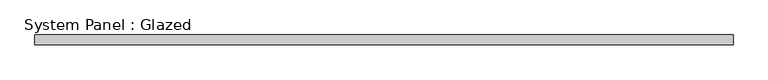
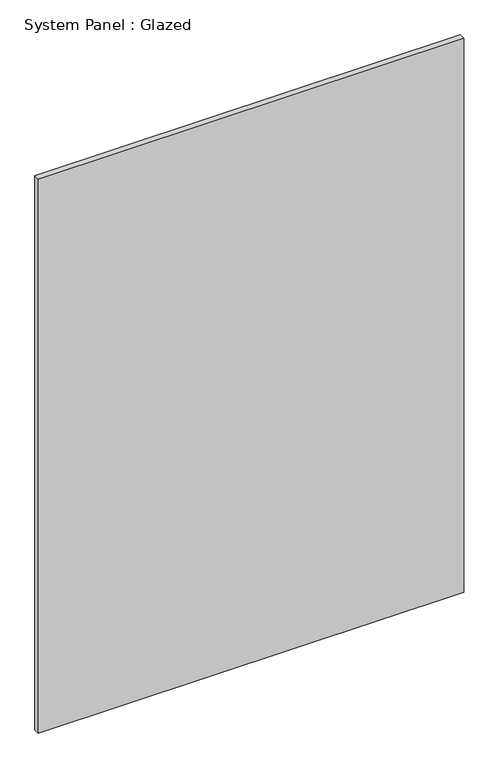
"""IFC4 building model written with IfcOpenShell, lengths in millimetres: plate geometry, System Panel : Glazed."""

import ifcopenshell
import ifcopenshell.guid

model = None  # the IFC model being written
_history = None  # IfcOwnerHistory: only IFC2X3 demands one
_inside = {}  # id of a spatial element -> (the spatial element, [elements in it])
_under = {}  # id of a project, library or spatial element -> (it, [spatial elements below it])
_declared = {}  # id of a project -> (the project, [libraries it declares])
_typed = {}  # id of a type object -> (the type object, [elements of that type])
_made_of = {}  # id of a material, layer set ... -> (it, [elements and type objects made of it])


def new_model(schema):
    """Start an empty IFC model of exactly this schema.

    Asked for "IFC4X3", IfcOpenShell would pick the latest addendum, in which some entities
    have other attributes; the version numbers below select the first issue.
    IFC2X3 requires an IfcOwnerHistory on every rooted entity: one is made here for all.
    """
    global model, _history
    if schema == "IFC4X3":
        model = ifcopenshell.file(schema_version=(4, 3, 0, 0))
    else:
        model = ifcopenshell.file(schema=schema)
    _inside.clear()
    _under.clear()
    _declared.clear()
    _typed.clear()
    _made_of.clear()
    _history = None
    if model.schema == "IFC2X3":
        org = make("IfcOrganization", Name="unknown")
        user = make(
            "IfcPersonAndOrganization",
            ThePerson=make("IfcPerson", FamilyName="unknown"),
            TheOrganization=org,
        )
        app = make(
            "IfcApplication",
            ApplicationDeveloper=org,
            Version="unknown",
            ApplicationFullName="unknown",
            ApplicationIdentifier="unknown",
        )
        _history = make(
            "IfcOwnerHistory",
            OwningUser=user,
            OwningApplication=app,
            ChangeAction="ADDED",
            CreationDate=0,
        )
    return model


def make(cls, **values):
    """One entity of the class cls with the attributes given. An attribute that is None is left unset."""
    return model.create_entity(
        cls, **{name: value for name, value in values.items() if value is not None}
    )


def rooted(cls, **values):
    """An entity with a GlobalId (a new one), such as an element, a storey or a relation."""
    return make(cls, GlobalId=ifcopenshell.guid.new(), OwnerHistory=_history, **values)


def si_unit(unit_type, name, prefix=None):
    """IfcSIUnit, for example si_unit("LENGTHUNIT", "METRE", prefix="MILLI")."""
    return make("IfcSIUnit", UnitType=unit_type, Prefix=prefix, Name=name)


def assignment(units):
    """IfcUnitAssignment: the units of a project."""
    return None if units is None else make("IfcUnitAssignment", Units=units)


def point(xyz):
    """IfcCartesianPoint."""
    return None if xyz is None else make("IfcCartesianPoint", Coordinates=xyz)


def direction(xyz):
    """IfcDirection."""
    return None if xyz is None else make("IfcDirection", DirectionRatios=xyz)


def frame(location, z_axis=None, x_axis=None):
    """IfcAxis2Placement3D, a coordinate frame: its origin and axes. An axis left out is left unset."""
    return make(
        "IfcAxis2Placement3D",
        Location=point(location),
        Axis=direction(z_axis),
        RefDirection=direction(x_axis),
    )


def origin():
    """The frame at (0, 0, 0) with its axes left unset."""
    return frame((0.0, 0.0, 0.0))


def origin_with_axes():
    """The frame at (0, 0, 0) with the z axis (0, 0, 1) and the x axis (1, 0, 0) written out."""
    return frame((0.0, 0.0, 0.0), z_axis=(0.0, 0.0, 1.0), x_axis=(1.0, 0.0, 0.0))


def place(relative_to, where):
    """IfcLocalPlacement: puts the frame where relative to a parent placement (None: the world)."""
    return make(
        "IfcLocalPlacement", PlacementRelTo=relative_to, RelativePlacement=where
    )


def context(
    kind, dimensions, precision=None, world=None, true_north=None, identifier=None
):
    """IfcGeometricRepresentationContext, for example the 3D "Model" context."""
    return make(
        "IfcGeometricRepresentationContext",
        ContextIdentifier=identifier,
        ContextType=kind,
        CoordinateSpaceDimension=dimensions,
        Precision=precision,
        WorldCoordinateSystem=world,
        TrueNorth=true_north,
    )


def project(units=None, contexts=None):
    """IfcProject with its units and contexts."""
    return rooted(
        "IfcProject",
        Name="project",
        RepresentationContexts=contexts,
        UnitsInContext=assignment(units),
    )


def spatial(cls, under=None, at=None, **own):
    """A site, building, storey or space (cls), placed at a placement, below another one or the project."""
    s = rooted(cls, ObjectPlacement=at, **own)
    if under is not None:
        _under.setdefault(under.id(), (under, []))[1].append(s)
    return s


def polyline(points):
    """IfcPolyline through the points."""
    return make("IfcPolyline", Points=[point(p) for p in points])


def outline(outer, holes=None, kind="AREA"):
    """IfcArbitraryClosedProfileDef: a profile drawn as a closed curve; with holes, ...WithVoids."""
    if holes is None:
        return make("IfcArbitraryClosedProfileDef", ProfileType=kind, OuterCurve=outer)
    return make(
        "IfcArbitraryProfileDefWithVoids",
        ProfileType=kind,
        OuterCurve=outer,
        InnerCurves=holes,
    )


def extrude(swept, where, along, depth):
    """IfcExtrudedAreaSolid: the profile swept, set in the frame where, extruded along a direction by depth."""
    return make(
        "IfcExtrudedAreaSolid",
        SweptArea=swept,
        Position=where,
        ExtrudedDirection=direction(along),
        Depth=depth,
    )


def shape(context_of_items, identifier, shape_type, items):
    """IfcShapeRepresentation: the items that make up one representation, for example the "Body"."""
    return make(
        "IfcShapeRepresentation",
        ContextOfItems=context_of_items,
        RepresentationIdentifier=identifier,
        RepresentationType=shape_type,
        Items=items,
    )


def source(mapping_origin, context_of_items, identifier, shape_type, items):
    """IfcRepresentationMap: a shape defined once, which mapped items show again and again."""
    return make(
        "IfcRepresentationMap",
        MappingOrigin=mapping_origin,
        MappedRepresentation=shape(context_of_items, identifier, shape_type, items),
    )


def transform(
    local_origin,
    x_axis=None,
    y_axis=None,
    z_axis=None,
    scale=None,
    scale2=None,
    scale3=None,
    uniform=True,
):
    """IfcCartesianTransformationOperator3D, or its non-uniform kind. x_axis, y_axis, z_axis: its Axis1, 2, 3."""
    if uniform:
        return make(
            "IfcCartesianTransformationOperator3D",
            Axis1=direction(x_axis),
            Axis2=direction(y_axis),
            LocalOrigin=point(local_origin),
            Scale=scale,
            Axis3=direction(z_axis),
        )
    return make(
        "IfcCartesianTransformationOperator3DnonUniform",
        Axis1=direction(x_axis),
        Axis2=direction(y_axis),
        LocalOrigin=point(local_origin),
        Scale=scale,
        Axis3=direction(z_axis),
        Scale2=scale2,
        Scale3=scale3,
    )


def mapped(mapping_source, mapping_target):
    """IfcMappedItem: shows the shape of a source again, moved by a transform."""
    return make(
        "IfcMappedItem", MappingSource=mapping_source, MappingTarget=mapping_target
    )


def made_of(thing, what):
    """Note that an element or type object is made of a material, layer set ...; save() writes the relation."""
    if what is not None:
        _made_of.setdefault(what.id(), (what, []))[1].append(thing)
    return thing


def element(
    cls,
    number,
    at=None,
    inside=None,
    cuts=None,
    type_object=None,
    material=None,
    context=None,
    identifier="Body",
    shape_type=None,
    held_by="IfcProductDefinitionShape",
    body=None,
    shapes=None,
    **own,
):
    """One element of the class cls, such as IfcWall. Its Tag is "e" and its number.

    at: its placement. inside: the storey or other place that contains it. cuts: it is an
    opening in that element (IfcRelVoidsElement). A single representation is given by context,
    identifier, shape_type and body (its items); several are given by shapes. held_by: the class
    of the entity that holds the representations. save() writes the other relations.
    """
    e = rooted(cls, Tag="e%d" % number, ObjectPlacement=at, **own)
    if body is not None:
        shapes = [shape(context, identifier, shape_type, body)]
    if shapes is not None:
        e.Representation = make(held_by, Representations=shapes)
    if inside is not None:
        _inside.setdefault(inside.id(), (inside, []))[1].append(e)
    if cuts is not None:
        rooted(
            "IfcRelVoidsElement", RelatingBuildingElement=cuts, RelatedOpeningElement=e
        )
    if type_object is not None:
        _typed.setdefault(type_object.id(), (type_object, []))[1].append(e)
    return made_of(e, material)


def aggregate(whole, parts):
    """IfcRelAggregates: a whole, such as a stair, and the parts it consists of."""
    return rooted("IfcRelAggregates", RelatingObject=whole, RelatedObjects=parts)


def save(model, path):
    """Write the relations noted so far, then the file.

    IfcRelAggregates (storeys below a building ...), IfcRelContainedInSpatialStructure (elements
    in a storey), IfcRelDefinesByType, IfcRelAssociatesMaterial and IfcRelDeclares: one each for
    every whole, place, type object, material and project.
    """
    for whole, parts in _under.values():
        aggregate(whole, parts)
    for where, things in _inside.values():
        rooted(
            "IfcRelContainedInSpatialStructure",
            RelatedElements=things,
            RelatingStructure=where,
        )
    for kind, things in _typed.values():
        rooted("IfcRelDefinesByType", RelatedObjects=things, RelatingType=kind)
    for what, things in _made_of.values():
        rooted("IfcRelAssociatesMaterial", RelatedObjects=things, RelatingMaterial=what)
    for by, libraries in _declared.values():
        rooted("IfcRelDeclares", RelatingContext=by, RelatedDefinitions=libraries)
    model.write(path)


def system_panel_glazed_55ebe308(model_context):
    return source(origin(), model_context, "Body", "SweptSolid", [
        extrude(outline(polyline([(890.0, -49.5), (-890.0, -49.5), (-890.0, -24.5), (890.0, -24.5), (890.0, -49.5)])), origin_with_axes(), (0.0, 0.0, 1.0), 2450.0),
    ])


if __name__ == "__main__":
    model = new_model("IFC4")
    model_context = context("Model", 3, world=origin())
    ifc_project = project(units=[si_unit("LENGTHUNIT", "METRE", prefix="MILLI")], contexts=[model_context])
    site = spatial("IfcSite", under=ifc_project)
    building = spatial("IfcBuilding", under=site)
    placement = place(None, origin())
    system_panel_glazed_shape = system_panel_glazed_55ebe308(model_context)
    element("IfcPlate", 1, ObjectType="System Panel : Glazed", at=placement, inside=building, context=model_context, shape_type="MappedRepresentation", body=[
        mapped(system_panel_glazed_shape, transform((0.0, 0.0, 0.0), x_axis=(1.0, 0.0, 0.0), y_axis=(0.0, 1.0, 0.0), z_axis=(0.0, 0.0, 1.0))),
    ])
    save(model, "model.ifc")

# Revit data of these elements
# Type "System Panel : Glazed"
#   Keynote = "H11"
#   Construction Type Id = "GSP4R"
#   Analytic Construction = "1/8 in Pilkington single glazing"
#   Visual Light Transmittance = 0.9
#   Solar Heat Gain Coefficient = 0.86
#   Heat Transfer Coefficient (U) = 6.7069 W/(m²·K)
# Element 1 (IfcPlate, "System Panel : Glazed")
#   Materials on its faces: "Glass"
# Materials
#   "Glass": class "Glass", colour RGB 0 128 192, transparency 0.9, Description = "Soda Lime Glass", Cost = 0
